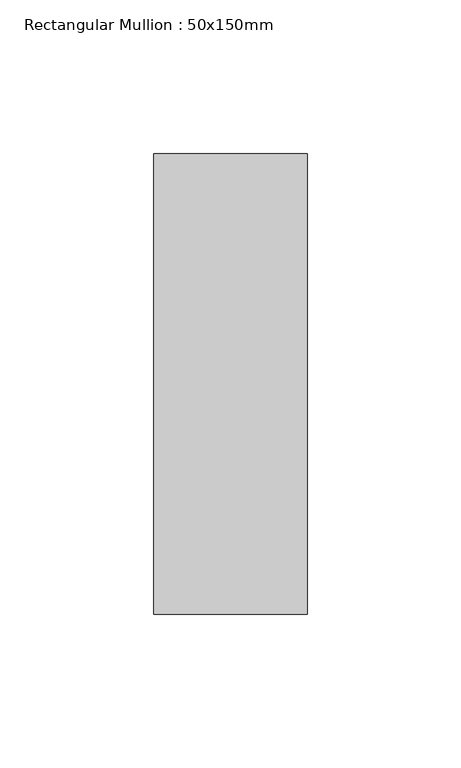
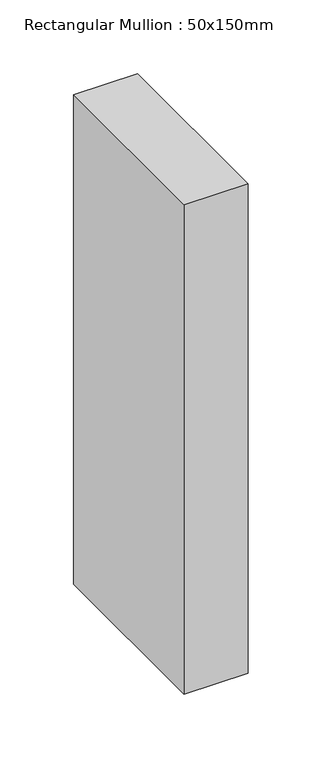
"""IFC4 building model written with IfcOpenShell, lengths in millimetres: member geometry, Rectangular Mullion : 50x150mm."""

from ifc_helpers import new_model, si_unit, frame, origin, place, context, project, spatial, polyline, outline, extrude, source, transform, mapped, element, save


def rectangular_mullion_50x150mm_ee1a5559(model_context):
    return source(origin(), model_context, "Body", "SweptSolid", [
        extrude(outline(polyline([(0.0, 75.0), (0.0, -75.0), (-50.0, -75.0), (-50.0, 75.0), (0.0, 75.0)])), frame((0.0, 0.0, -404.9999998), z_axis=(0.0, 0.0, 1.0), x_axis=(1.0, 0.0, 0.0)), (0.0, 0.0, 1.0), 404.9999998),
    ])


if __name__ == "__main__":
    model = new_model("IFC4")
    model_context = context("Model", 3, world=origin())
    ifc_project = project(units=[si_unit("LENGTHUNIT", "METRE", prefix="MILLI")], contexts=[model_context])
    site = spatial("IfcSite", under=ifc_project)
    building = spatial("IfcBuilding", under=site)
    placement = place(None, origin())
    rectangular_mullion_50x150mm_shape = rectangular_mullion_50x150mm_ee1a5559(model_context)
    element("IfcMember", 1, ObjectType="Rectangular Mullion : 50x150mm", at=placement, inside=building, context=model_context, shape_type="MappedRepresentation", body=[
        mapped(rectangular_mullion_50x150mm_shape, transform((0.0, 0.0, 0.0), x_axis=(1.0, 0.0, 0.0), y_axis=(0.0, 1.0, 0.0), z_axis=(0.0, 0.0, 1.0))),
    ])
    save(model, "model.ifc")

# Revit data of these elements
# Type "Rectangular Mullion : 50x150mm"
#   Keynote = "H11"
#   built-in parameter 1007304 = 0.492126 (stored number, unit not read)
#   built-in parameter 1007301 = 0.082021 (stored number, unit not read)
#   built-in parameter 1007300 = 0.082021 (stored number, unit not read)
# Element 1 (IfcMember, "Rectangular Mullion : 50x150mm")
#   Materials on its faces: "Aluminium"
# Materials
#   "Aluminium": class "Metal", colour RGB 247 247 247, transparency 0, Description = "Aluminium 6061", Cost = 0
